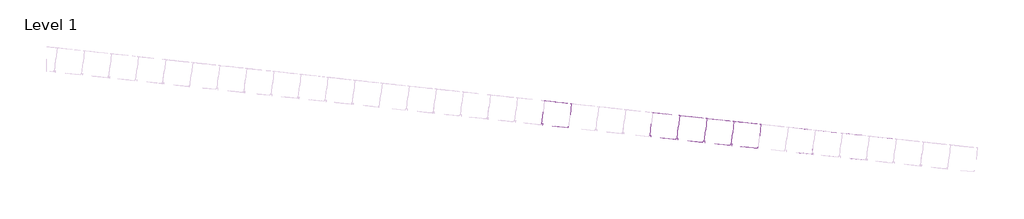
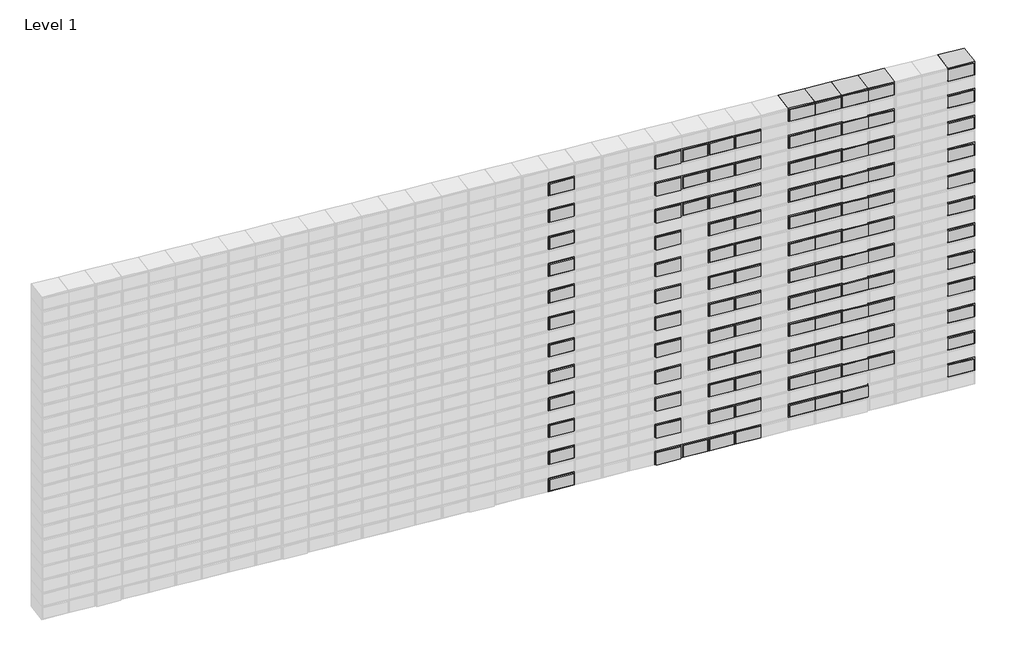
# One storey, part 17 of 18: 111 proxies.
# Revit data of these elements (continued)
# Elements 36, 37, 38, 39, 40, 41, 42, 43, 44, 45, 46, 47, 48, 49, 50, 51, 52, 53, 54, 55, 56, 57, 58, 59 (IfcBuildingElementProxy, "00_GMA_steen_versie_6 : Geel") (continued)
#   Phase Created = New Construction
#   Materials on its faces: "20_voeg", "21_steen_geel"
# Elements 60, 61, 62, 63, 64, 65, 66, 67, 68, 69, 70, 71, 72, 73, 74, 75, 76, 77, 78, 79, 80, 81, 82, 83, 84, 85, 86, 87, 88, 89, 90, 91, 92, 93, 94, 95, 96, 97, 98, 99 (IfcBuildingElementProxy, "00_GMA_steen_versie_6 : Rood")
#   StootvoegLinksHalfOnder = 5 mm
#   StootvoegLinksHalfBoven = 5 mm
#   StootVoegRechtsHalfOnder = 5 mm
#   StootVoegRechtsHalfBoven = 5 mm
#   StootVoegBreedteRechts = 10 mm
#   StootVoegBreedteLinks = 10 mm
#   LintVoegOnderHalf = 5 mm
#   LintVoegOnder = 10 mm
#   LintVoegBovenHalf = 5 mm
#   LintVoegBoven = 10 mm
#   Phase Created = New Construction
#   Materials on its faces: "20_voeg", "21_steen_rood"
# Elements 100, 101, 102, 103, 104, 105, 106, 107, 108, 109, 110, 111 (IfcBuildingElementProxy, "00_GMA_steen_versie_6 : Rood")
#   StootvoegLinksHalfOnder = 5 mm
#   StootvoegLinksHalfBoven = 5 mm
#   StootVoegRechtsHalfOnder = 5 mm
#   StootVoegRechtsHalfBoven = 5 mm
#   StootVoegBreedteRechts = 10 mm
#   StootVoegBreedteLinks = 10 mm
#   LintVoegOnderHalf = 0 mm
#   LintVoegOnder = 0 mm
#   LintVoegBovenHalf = 5 mm
#   LintVoegBoven = 10 mm
#   Phase Created = New Construction
#   Materials on its faces: "20_voeg", "21_steen_rood"
# Materials
#   "21_steen_geel": class "Unassigned", colour RGB 202 202 0, transparency 0, Cost = 0
#   "20_voeg": class "Concrete", colour RGB 86 86 86, transparency 0, Manufacturer = "RevitGG", URL = "www.revitgg.nl", Description = "zandcement, generiek materiaal", Cost = 0
#   "21_steen_rood": class "Unassigned", colour RGB 213 111 43, transparency 0, Cost = 0
